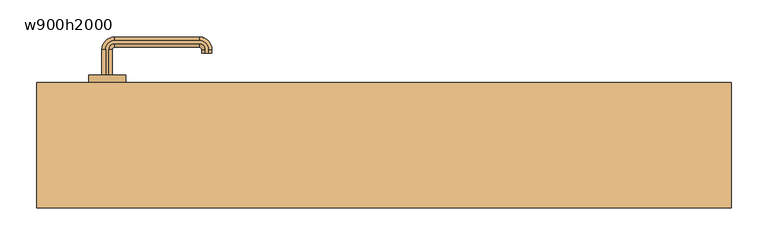
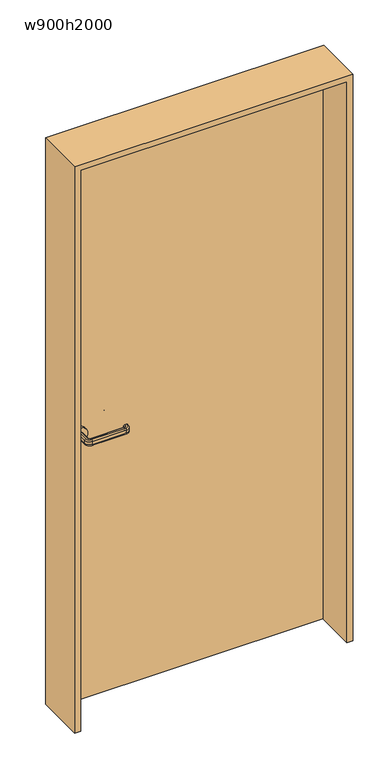
"""IFC4 building model written with IfcOpenShell, lengths in millimetres: door geometry, 片開き : w900h2000."""

from ifc_helpers import new_model, si_unit, point, frame, frame_2d, origin, origin_with_axes, place, context, project, spatial, polyline, circle_curve, ellipse_curve, trimmed, segment, composite_curve, outline, extrude, source, transform, mapped, element, save
from ifc_brep_helpers import plane_surface, cylinder_surface, revolved_surface, advanced_brep


def w900h2000_7a121c74(model_context):
    return source(origin(), model_context, "Body", "SolidModel", [
        advanced_brep(
        [(-377.0, 95.0, 960.0), (-382.0, 95.0, 955.0), (-382.0, 95.0, 945.0477623), (-377.0, 95.0, 940.0477623), (-373.0, 95.0, 940.0477623), (-368.0, 95.0, 945.0477623), (-368.0, 95.0, 955.0), (-373.0, 95.0, 960.0), (-377.0, 130.0, 960.0), (-382.0, 130.0, 955.0), (-382.0, 130.0, 945.0477623), (-377.0, 130.0, 940.0477623), (-365.0, 142.0, 940.0477623), (-250.0, 142.0, 940.0477623), (-238.0, 130.0, 940.0477623), (-238.0, 125.0, 940.0477623), (-242.0, 125.0, 940.0477623), (-242.0, 130.0, 940.0477623), (-250.0, 138.0, 940.0477623), (-365.0, 138.0, 940.0477623), (-373.0, 130.0, 940.0477623), (-368.0, 130.0, 945.0477623), (-368.0, 130.0, 955.0), (-373.0, 130.0, 960.0), (-365.0, 138.0, 960.0), (-250.0, 138.0, 960.0), (-242.0, 130.0, 960.0), (-242.0, 125.0, 960.0), (-238.0, 125.0, 960.0), (-238.0, 130.0, 960.0), (-250.0, 142.0, 960.0), (-365.0, 142.0, 960.0), (-365.0, 147.0, 955.0), (-365.0, 147.0, 945.0477623), (-365.0, 133.0, 945.0477623), (-365.0, 133.0, 955.0), (-250.0, 147.0, 955.0), (-250.0, 147.0, 945.0477623), (-250.0, 133.0, 945.0477623), (-250.0, 133.0, 955.0), (-233.0, 130.0, 955.0), (-233.0, 130.0, 945.0477623), (-247.0, 130.0, 945.0477623), (-247.0, 130.0, 955.0), (-247.0, 125.0, 955.0), (-247.0, 125.0, 945.0477623), (-233.0, 125.0, 945.0477623), (-233.0, 125.0, 955.0)],
        [
            (0, 1, circle_curve(frame((-377.0, 95.0, 955.0), z_axis=(0.0, -1.0, 0.0), x_axis=(-1.0, 0.0, 0.0)), 5.0)),
            (1, 2),
            (2, 3, circle_curve(frame((-377.0, 95.0, 945.0477623), z_axis=(0.0, -1.0, 0.0), x_axis=(-1.0, 0.0, 0.0)), 5.0)),
            (3, 4),
            (4, 5, circle_curve(frame((-373.0, 95.0, 945.0477623), z_axis=(0.0, -1.0, 0.0), x_axis=(-1.0, 0.0, 0.0)), 5.0)),
            (5, 6),
            (6, 7, circle_curve(frame((-373.0, 95.0, 955.0), z_axis=(0.0, -1.0, 0.0), x_axis=(-1.0, 0.0, 0.0)), 5.0)),
            (7, 0),
            (0, 8),
            (8, 9, circle_curve(frame((-377.0, 130.0, 955.0), z_axis=(0.0, -1.0, 0.0), x_axis=(-1.0, 0.0, 0.0)), 5.0)),
            (9, 1),
            (9, 10),
            (10, 2),
            (10, 11, circle_curve(frame((-377.0, 130.0, 945.0477623), z_axis=(0.0, -1.0, 0.0), x_axis=(-1.0, 0.0, 0.0)), 5.0)),
            (11, 3),
            (11, 12, circle_curve(frame((-365.0, 130.0, 940.0477623), z_axis=(0.0, 0.0, -1.0), x_axis=(-1.0, 0.0, 0.0)), 12.0)),
            (12, 13),
            (13, 14, circle_curve(frame((-250.0, 130.0, 940.0477623), z_axis=(0.0, 0.0, -1.0), x_axis=(0.0, 1.0, 0.0)), 12.0)),
            (14, 15),
            (15, 16),
            (16, 17),
            (17, 18, circle_curve(frame((-250.0, 130.0, 940.0477623), z_axis=(0.0, 0.0, 1.0), x_axis=(0.0, 1.0, 0.0)), 8.0)),
            (18, 19),
            (19, 20, circle_curve(frame((-365.0, 130.0, 940.0477623), z_axis=(0.0, 0.0, 1.0), x_axis=(-1.0, 0.0, 0.0)), 8.0)),
            (20, 4),
            (20, 21, circle_curve(frame((-373.0, 130.0, 945.0477623), z_axis=(0.0, -1.0, 0.0), x_axis=(-1.0, 0.0, 0.0)), 5.0)),
            (21, 5),
            (21, 22),
            (22, 6),
            (22, 23, circle_curve(frame((-373.0, 130.0, 955.0), z_axis=(0.0, -1.0, 0.0), x_axis=(-1.0, 0.0, 0.0)), 5.0)),
            (23, 7),
            (23, 24, circle_curve(frame((-365.0, 130.0, 960.0), z_axis=(0.0, 0.0, -1.0), x_axis=(-1.0, 0.0, 0.0)), 8.0)),
            (24, 25),
            (25, 26, circle_curve(frame((-250.0, 130.0, 960.0), z_axis=(0.0, 0.0, -1.0), x_axis=(0.0, 1.0, 0.0)), 8.0)),
            (26, 27),
            (27, 28),
            (28, 29),
            (29, 30, circle_curve(frame((-250.0, 130.0, 960.0), z_axis=(0.0, 0.0, 1.0), x_axis=(0.0, 1.0, 0.0)), 12.0)),
            (30, 31),
            (31, 8, circle_curve(frame((-365.0, 130.0, 960.0), z_axis=(0.0, 0.0, 1.0), x_axis=(-1.0, 0.0, 0.0)), 12.0)),
            (32, 9, circle_curve(frame((-365.0, 130.0, 955.0), z_axis=(0.0, 0.0, 1.0), x_axis=(-1.0, 0.0, 0.0)), 17.0)),
            (31, 32, circle_curve(frame((-365.0, 142.0, 955.0), z_axis=(-1.0, 0.0, 0.0), x_axis=(0.0, 1.0, 0.0)), 5.0)),
            (33, 10, circle_curve(frame((-365.0, 130.0, 945.0477623), z_axis=(0.0, 0.0, 1.0), x_axis=(-1.0, 0.0, 0.0)), 17.0)),
            (32, 33),
            (33, 12, circle_curve(frame((-365.0, 142.0, 945.0477623), z_axis=(-1.0, 0.0, 0.0), x_axis=(0.0, 1.0, 0.0)), 5.0)),
            (34, 21, circle_curve(frame((-365.0, 130.0, 945.0477623), z_axis=(0.0, 0.0, 1.0), x_axis=(-1.0, 0.0, 0.0)), 3.0)),
            (19, 34, circle_curve(frame((-365.0, 138.0, 945.0477623), z_axis=(-1.0, 0.0, 0.0), x_axis=(0.0, 1.0, 0.0)), 5.0)),
            (35, 22, circle_curve(frame((-365.0, 130.0, 955.0), z_axis=(0.0, 0.0, 1.0), x_axis=(-1.0, 0.0, 0.0)), 3.0)),
            (34, 35),
            (35, 24, circle_curve(frame((-365.0, 138.0, 955.0), z_axis=(-1.0, 0.0, 0.0), x_axis=(0.0, 1.0, 0.0)), 5.0)),
            (30, 36, circle_curve(frame((-250.0, 142.0, 955.0), z_axis=(-1.0, 0.0, 0.0), x_axis=(0.0, 1.0, 0.0)), 5.0)),
            (36, 32),
            (36, 37),
            (37, 33),
            (37, 13, circle_curve(frame((-250.0, 142.0, 945.0477623), z_axis=(-1.0, 0.0, 0.0), x_axis=(0.0, 1.0, 0.0)), 5.0)),
            (18, 38, circle_curve(frame((-250.0, 138.0, 945.0477623), z_axis=(-1.0, 0.0, 0.0), x_axis=(0.0, 1.0, 0.0)), 5.0)),
            (38, 34),
            (38, 39),
            (39, 35),
            (39, 25, circle_curve(frame((-250.0, 138.0, 955.0), z_axis=(-1.0, 0.0, 0.0), x_axis=(0.0, 1.0, 0.0)), 5.0)),
            (40, 36, circle_curve(frame((-250.0, 130.0, 955.0), z_axis=(0.0, 0.0, 1.0), x_axis=(0.0, 1.0, 0.0)), 17.0)),
            (29, 40, circle_curve(frame((-238.0, 130.0, 955.0), z_axis=(0.0, 1.0, 0.0), x_axis=(1.0, 0.0, 0.0)), 5.0)),
            (41, 37, circle_curve(frame((-250.0, 130.0, 945.0477623), z_axis=(0.0, 0.0, 1.0), x_axis=(0.0, 1.0, 0.0)), 17.0)),
            (40, 41),
            (41, 14, circle_curve(frame((-238.0, 130.0, 945.0477623), z_axis=(0.0, 1.0, 0.0), x_axis=(1.0, 0.0, 0.0)), 5.0)),
            (42, 38, circle_curve(frame((-250.0, 130.0, 945.0477623), z_axis=(0.0, 0.0, 1.0), x_axis=(0.0, 1.0, 0.0)), 3.0)),
            (17, 42, circle_curve(frame((-242.0, 130.0, 945.0477623), z_axis=(0.0, 1.0, 0.0), x_axis=(1.0, 0.0, 0.0)), 5.0)),
            (43, 39, circle_curve(frame((-250.0, 130.0, 955.0), z_axis=(0.0, 0.0, 1.0), x_axis=(0.0, 1.0, 0.0)), 3.0)),
            (42, 43),
            (43, 26, circle_curve(frame((-242.0, 130.0, 955.0), z_axis=(0.0, 1.0, 0.0), x_axis=(1.0, 0.0, 0.0)), 5.0)),
            (27, 44, circle_curve(frame((-242.0, 125.0, 955.0), z_axis=(0.0, -1.0, 0.0), x_axis=(1.0, 0.0, 0.0)), 5.0)),
            (44, 45),
            (45, 16, circle_curve(frame((-242.0, 125.0, 945.0477623), z_axis=(0.0, -1.0, 0.0), x_axis=(1.0, 0.0, 0.0)), 5.0)),
            (15, 46, circle_curve(frame((-238.0, 125.0, 945.0477623), z_axis=(0.0, -1.0, 0.0), x_axis=(1.0, 0.0, 0.0)), 5.0)),
            (46, 47),
            (47, 28, circle_curve(frame((-238.0, 125.0, 955.0), z_axis=(0.0, -1.0, 0.0), x_axis=(1.0, 0.0, 0.0)), 5.0)),
            (47, 40),
            (46, 41),
            (45, 42),
            (44, 43),
        ],
        [
            plane_surface(frame((-385.198039, 95.0, 950.0), z_axis=(0.0, -1.0, 0.0), x_axis=(0.0, 0.0, 1.0))),
            cylinder_surface(frame((-377.0, 95.0, 955.0), z_axis=(0.0, -1.0, 0.0), x_axis=(-1.0, 0.0, 0.0)), 5.0),
            plane_surface(frame((-382.0, 95.0, 955.0), z_axis=(-1.0, 0.0, 0.0), x_axis=(0.0, 1.0, 0.0))),
            cylinder_surface(frame((-377.0, 95.0, 945.0477623), z_axis=(0.0, -1.0, 0.0), x_axis=(-1.0, 0.0, 0.0)), 5.0),
            plane_surface(frame((-377.0, 95.0, 940.0477623), z_axis=(0.0, 0.0, -1.0), x_axis=(0.0, 1.0, 0.0))),
            cylinder_surface(frame((-373.0, 95.0, 945.0477623), z_axis=(0.0, -1.0, 0.0), x_axis=(-1.0, 0.0, 0.0)), 5.0),
            plane_surface(frame((-368.0, 95.0, 945.0477623), z_axis=(1.0, 0.0, 0.0), x_axis=(0.0, 1.0, 0.0))),
            cylinder_surface(frame((-373.0, 95.0, 955.0), z_axis=(0.0, -1.0, 0.0), x_axis=(-1.0, 0.0, 0.0)), 5.0),
            plane_surface(frame((-373.0, 95.0, 960.0), z_axis=(0.0, 0.0, 1.0), x_axis=(0.0, 1.0, 0.0))),
            revolved_surface(trimmed(ellipse_curve(frame((-377.0, 130.0, 955.0), z_axis=(0.0, -1.0, 0.0), x_axis=(-1.0, 0.0, 0.0)), 5.0, 5.0), [point((-377.0, 130.0, 960.0))], [point((-382.0, 130.0, 955.0))], True, "CARTESIAN"), (-365.0, 130.0, 950.0), (0.0, 0.0, -1.0)),
            cylinder_surface(frame((-365.0, 130.0, 950.0), z_axis=(0.0, 0.0, -1.0), x_axis=(-1.0, 0.0, 0.0)), 17.0),
            revolved_surface(trimmed(ellipse_curve(frame((-377.0, 130.0, 945.0477623), z_axis=(0.0, -1.0, 0.0), x_axis=(-1.0, 0.0, 0.0)), 5.0, 5.0), [point((-382.0, 130.0, 945.0477623))], [point((-377.0, 130.0, 940.0477623))], True, "CARTESIAN"), (-365.0, 130.0, 950.0), (0.0, 0.0, -1.0)),
            revolved_surface(trimmed(ellipse_curve(frame((-373.0, 130.0, 945.0477623), z_axis=(0.0, -1.0, 0.0), x_axis=(-1.0, 0.0, 0.0)), 5.0, 5.0), [point((-373.0, 130.0, 940.0477623))], [point((-368.0, 130.0, 945.0477623))], True, "CARTESIAN"), (-365.0, 130.0, 950.0), (0.0, 0.0, -1.0)),
            revolved_surface(polyline([(-368.0, 130.0, 945.0477623), (-368.0, 130.0, 955.0)]), (-365.0, 130.0, 950.0), (0.0, 0.0, -1.0)),
            revolved_surface(trimmed(ellipse_curve(frame((-373.0, 130.0, 955.0), z_axis=(0.0, -1.0, 0.0), x_axis=(-1.0, 0.0, 0.0)), 5.0, 5.0), [point((-368.0, 130.0, 955.0))], [point((-373.0, 130.0, 960.0))], True, "CARTESIAN"), (-365.0, 130.0, 950.0), (0.0, 0.0, -1.0)),
            cylinder_surface(frame((-365.0, 142.0, 955.0), z_axis=(-1.0, 0.0, 0.0), x_axis=(0.0, 1.0, 0.0)), 5.0),
            plane_surface(frame((-365.0, 147.0, 955.0), z_axis=(0.0, 1.0, 0.0), x_axis=(1.0, 0.0, 0.0))),
            cylinder_surface(frame((-365.0, 142.0, 945.0477623), z_axis=(-1.0, 0.0, 0.0), x_axis=(0.0, 1.0, 0.0)), 5.0),
            cylinder_surface(frame((-365.0, 138.0, 945.0477623), z_axis=(-1.0, 0.0, 0.0), x_axis=(0.0, 1.0, 0.0)), 5.0),
            plane_surface(frame((-365.0, 133.0, 945.0477623), z_axis=(0.0, -1.0, 0.0), x_axis=(1.0, 0.0, 0.0))),
            cylinder_surface(frame((-365.0, 138.0, 955.0), z_axis=(-1.0, 0.0, 0.0), x_axis=(0.0, 1.0, 0.0)), 5.0),
            revolved_surface(trimmed(ellipse_curve(frame((-250.0, 142.0, 955.0), z_axis=(-1.0, 0.0, 0.0), x_axis=(0.0, 1.0, 0.0)), 5.0, 5.0), [point((-250.0, 142.0, 960.0))], [point((-250.0, 147.0, 955.0))], True, "CARTESIAN"), (-250.0, 130.0, 950.0), (0.0, 0.0, -1.0)),
            cylinder_surface(frame((-250.0, 130.0, 950.0), z_axis=(0.0, 0.0, -1.0), x_axis=(0.0, 1.0, 0.0)), 17.0),
            revolved_surface(trimmed(ellipse_curve(frame((-250.0, 142.0, 945.0477623), z_axis=(-1.0, 0.0, 0.0), x_axis=(0.0, 1.0, 0.0)), 5.0, 5.0), [point((-250.0, 147.0, 945.0477623))], [point((-250.0, 142.0, 940.0477623))], True, "CARTESIAN"), (-250.0, 130.0, 950.0), (0.0, 0.0, -1.0)),
            revolved_surface(trimmed(ellipse_curve(frame((-250.0, 138.0, 945.0477623), z_axis=(-1.0, 0.0, 0.0), x_axis=(0.0, 1.0, 0.0)), 5.0, 5.0), [point((-250.0, 138.0, 940.0477623))], [point((-250.0, 133.0, 945.0477623))], True, "CARTESIAN"), (-250.0, 130.0, 950.0), (0.0, 0.0, -1.0)),
            revolved_surface(polyline([(-250.0, 133.0, 945.0477623), (-250.0, 133.0, 955.0)]), (-250.0, 130.0, 950.0), (0.0, 0.0, -1.0)),
            revolved_surface(trimmed(ellipse_curve(frame((-250.0, 138.0, 955.0), z_axis=(-1.0, 0.0, 0.0), x_axis=(0.0, 1.0, 0.0)), 5.0, 5.0), [point((-250.0, 133.0, 955.0))], [point((-250.0, 138.0, 960.0))], True, "CARTESIAN"), (-250.0, 130.0, 950.0), (0.0, 0.0, -1.0)),
            plane_surface(frame((-250.198039, 125.0, 950.0), z_axis=(0.0, -1.0, 0.0), x_axis=(0.0, 0.0, -1.0))),
            cylinder_surface(frame((-238.0, 130.0, 955.0), z_axis=(0.0, 1.0, 0.0), x_axis=(1.0, 0.0, 0.0)), 5.0),
            plane_surface(frame((-233.0, 130.0, 955.0), z_axis=(1.0, 0.0, 0.0), x_axis=(0.0, -1.0, 0.0))),
            cylinder_surface(frame((-238.0, 130.0, 945.0477623), z_axis=(0.0, 1.0, 0.0), x_axis=(1.0, 0.0, 0.0)), 5.0),
            cylinder_surface(frame((-242.0, 130.0, 945.0477623), z_axis=(0.0, 1.0, 0.0), x_axis=(1.0, 0.0, 0.0)), 5.0),
            plane_surface(frame((-247.0, 130.0, 945.0477623), z_axis=(-1.0, 0.0, 0.0), x_axis=(0.0, -1.0, 0.0))),
            cylinder_surface(frame((-242.0, 130.0, 955.0), z_axis=(0.0, 1.0, 0.0), x_axis=(1.0, 0.0, 0.0)), 5.0),
        ],
        [
            (0, [[1, 2, 3, 4, 5, 6, 7, 8]]),
            (1, [[-1, 9, 10, 11]]),
            (2, [[-2, -11, 12, 13]]),
            (3, [[-3, -13, 14, 15]]),
            (4, [[-4, -15, 16, 17, 18, 19, 20, 21, 22, 23, 24, 25]]),
            (5, [[-5, -25, 26, 27]]),
            (6, [[-6, -27, 28, 29]]),
            (7, [[-7, -29, 30, 31]]),
            (8, [[-8, -31, 32, 33, 34, 35, 36, 37, 38, 39, 40, -9]]),
            (9, [[41, -10, -40, 42]]),
            (10, [[43, -12, -41, 44]]),
            (11, [[-16, -14, -43, 45]]),
            (12, [[46, -26, -24, 47]]),
            (13, [[48, -28, -46, 49]]),
            (14, [[-32, -30, -48, 50]]),
            (15, [[-42, -39, 51, 52]]),
            (16, [[-44, -52, 53, 54]]),
            (17, [[-45, -54, 55, -17]]),
            (18, [[-47, -23, 56, 57]]),
            (19, [[-49, -57, 58, 59]]),
            (20, [[-50, -59, 60, -33]]),
            (21, [[61, -51, -38, 62]]),
            (22, [[63, -53, -61, 64]]),
            (23, [[-18, -55, -63, 65]]),
            (24, [[66, -56, -22, 67]]),
            (25, [[68, -58, -66, 69]]),
            (26, [[-34, -60, -68, 70]]),
            (27, [[-36, 71, 72, 73, -20, 74, 75, 76]]),
            (28, [[-62, -37, -76, 77]]),
            (29, [[-64, -77, -75, 78]]),
            (30, [[-65, -78, -74, -19]]),
            (31, [[-67, -21, -73, 79]]),
            (32, [[-69, -79, -72, 80]]),
            (33, [[-70, -80, -71, -35]]),
        ],
    ),
        advanced_brep(
        [(-373.0, 45.0, 940.0), (-377.0, 45.0, 940.0), (-382.0, 45.0, 945.0), (-382.0, 45.0, 955.0), (-377.0, 45.0, 960.0), (-373.0, 45.0, 960.0), (-368.0, 45.0, 955.0), (-368.0, 45.0, 945.0), (-373.0, 10.0, 940.0), (-365.0, 2.0, 940.0), (-250.0, 2.0, 940.0), (-242.0, 10.0, 940.0), (-242.0, 15.0, 940.0), (-238.0, 15.0, 940.0), (-238.0, 10.0, 940.0), (-250.0, -2.0, 940.0), (-365.0, -2.0, 940.0), (-377.0, 10.0, 940.0), (-382.0, 10.0, 945.0), (-382.0, 10.0, 955.0), (-377.0, 10.0, 960.0), (-365.0, -2.0, 960.0), (-250.0, -2.0, 960.0), (-238.0, 10.0, 960.0), (-238.0, 15.0, 960.0), (-242.0, 15.0, 960.0), (-242.0, 10.0, 960.0), (-250.0, 2.0, 960.0), (-365.0, 2.0, 960.0), (-373.0, 10.0, 960.0), (-368.0, 10.0, 955.0), (-368.0, 10.0, 945.0), (-365.0, -7.0, 945.0), (-365.0, -7.0, 955.0), (-365.0, 7.0, 955.0), (-365.0, 7.0, 945.0), (-250.0, -7.0, 945.0), (-250.0, -7.0, 955.0), (-250.0, 7.0, 955.0), (-250.0, 7.0, 945.0), (-233.0, 10.0, 945.0), (-233.0, 10.0, 955.0), (-247.0, 10.0, 955.0), (-247.0, 10.0, 945.0), (-247.0, 15.0, 945.0), (-247.0, 15.0, 955.0), (-233.0, 15.0, 955.0), (-233.0, 15.0, 945.0)],
        [
            (0, 1),
            (1, 2, circle_curve(frame((-377.0, 45.0, 945.0), z_axis=(0.0, 1.0, 0.0), x_axis=(1.0, 0.0, 0.0)), 5.0)),
            (2, 3),
            (3, 4, circle_curve(frame((-377.0, 45.0, 955.0), z_axis=(0.0, 1.0, 0.0), x_axis=(1.0, 0.0, 0.0)), 5.0)),
            (4, 5),
            (5, 6, circle_curve(frame((-373.0, 45.0, 955.0), z_axis=(0.0, 1.0, 0.0), x_axis=(1.0, 0.0, 0.0)), 5.0)),
            (6, 7),
            (7, 0, circle_curve(frame((-373.0, 45.0, 945.0), z_axis=(0.0, 1.0, 0.0), x_axis=(1.0, 0.0, 0.0)), 5.0)),
            (0, 8),
            (8, 9, circle_curve(frame((-365.0, 10.0, 940.0), z_axis=(0.0, 0.0, 1.0), x_axis=(-1.0, 0.0, 0.0)), 8.0)),
            (9, 10),
            (10, 11, circle_curve(frame((-250.0, 10.0, 940.0), z_axis=(0.0, 0.0, 1.0), x_axis=(0.0, -1.0, 0.0)), 8.0)),
            (11, 12),
            (12, 13),
            (13, 14),
            (14, 15, circle_curve(frame((-250.0, 10.0, 940.0), z_axis=(0.0, 0.0, -1.0), x_axis=(0.0, -1.0, 0.0)), 12.0)),
            (15, 16),
            (16, 17, circle_curve(frame((-365.0, 10.0, 940.0), z_axis=(0.0, 0.0, -1.0), x_axis=(-1.0, 0.0, 0.0)), 12.0)),
            (17, 1),
            (17, 18, circle_curve(frame((-377.0, 10.0, 945.0), z_axis=(0.0, 1.0, 0.0), x_axis=(1.0, 0.0, 0.0)), 5.0)),
            (18, 2),
            (18, 19),
            (19, 3),
            (19, 20, circle_curve(frame((-377.0, 10.0, 955.0), z_axis=(0.0, 1.0, 0.0), x_axis=(1.0, 0.0, 0.0)), 5.0)),
            (20, 4),
            (20, 21, circle_curve(frame((-365.0, 10.0, 960.0), z_axis=(0.0, 0.0, 1.0), x_axis=(-1.0, 0.0, 0.0)), 12.0)),
            (21, 22),
            (22, 23, circle_curve(frame((-250.0, 10.0, 960.0), z_axis=(0.0, 0.0, 1.0), x_axis=(0.0, -1.0, 0.0)), 12.0)),
            (23, 24),
            (24, 25),
            (25, 26),
            (26, 27, circle_curve(frame((-250.0, 10.0, 960.0), z_axis=(0.0, 0.0, -1.0), x_axis=(0.0, -1.0, 0.0)), 8.0)),
            (27, 28),
            (28, 29, circle_curve(frame((-365.0, 10.0, 960.0), z_axis=(0.0, 0.0, -1.0), x_axis=(-1.0, 0.0, 0.0)), 8.0)),
            (29, 5),
            (29, 30, circle_curve(frame((-373.0, 10.0, 955.0), z_axis=(0.0, 1.0, 0.0), x_axis=(1.0, 0.0, 0.0)), 5.0)),
            (30, 6),
            (30, 31),
            (31, 7),
            (31, 8, circle_curve(frame((-373.0, 10.0, 945.0), z_axis=(0.0, 1.0, 0.0), x_axis=(1.0, 0.0, 0.0)), 5.0)),
            (32, 18, circle_curve(frame((-365.0, 10.0, 945.0), z_axis=(0.0, 0.0, -1.0), x_axis=(-1.0, 0.0, 0.0)), 17.0)),
            (16, 32, circle_curve(frame((-365.0, -2.0, 945.0), z_axis=(-1.0, 0.0, 0.0), x_axis=(0.0, 1.0, 0.0)), 5.0)),
            (33, 19, circle_curve(frame((-365.0, 10.0, 955.0), z_axis=(0.0, 0.0, -1.0), x_axis=(-1.0, 0.0, 0.0)), 17.0)),
            (32, 33),
            (33, 21, circle_curve(frame((-365.0, -2.0, 955.0), z_axis=(-1.0, 0.0, 0.0), x_axis=(0.0, 1.0, 0.0)), 5.0)),
            (34, 30, circle_curve(frame((-365.0, 10.0, 955.0), z_axis=(0.0, 0.0, -1.0), x_axis=(-1.0, 0.0, 0.0)), 3.0)),
            (28, 34, circle_curve(frame((-365.0, 2.0, 955.0), z_axis=(-1.0, 0.0, 0.0), x_axis=(0.0, 1.0, 0.0)), 5.0)),
            (35, 31, circle_curve(frame((-365.0, 10.0, 945.0), z_axis=(0.0, 0.0, -1.0), x_axis=(-1.0, 0.0, 0.0)), 3.0)),
            (34, 35),
            (35, 9, circle_curve(frame((-365.0, 2.0, 945.0), z_axis=(-1.0, 0.0, 0.0), x_axis=(0.0, 1.0, 0.0)), 5.0)),
            (15, 36, circle_curve(frame((-250.0, -2.0, 945.0), z_axis=(-1.0, 0.0, 0.0), x_axis=(0.0, 1.0, 0.0)), 5.0)),
            (36, 32),
            (36, 37),
            (37, 33),
            (37, 22, circle_curve(frame((-250.0, -2.0, 955.0), z_axis=(-1.0, 0.0, 0.0), x_axis=(0.0, 1.0, 0.0)), 5.0)),
            (27, 38, circle_curve(frame((-250.0, 2.0, 955.0), z_axis=(-1.0, 0.0, 0.0), x_axis=(0.0, 1.0, 0.0)), 5.0)),
            (38, 34),
            (38, 39),
            (39, 35),
            (39, 10, circle_curve(frame((-250.0, 2.0, 945.0), z_axis=(-1.0, 0.0, 0.0), x_axis=(0.0, 1.0, 0.0)), 5.0)),
            (40, 36, circle_curve(frame((-250.0, 10.0, 945.0), z_axis=(0.0, 0.0, -1.0), x_axis=(0.0, -1.0, 0.0)), 17.0)),
            (14, 40, circle_curve(frame((-238.0, 10.0, 945.0), z_axis=(0.0, -1.0, 0.0), x_axis=(-1.0, 0.0, 0.0)), 5.0)),
            (41, 37, circle_curve(frame((-250.0, 10.0, 955.0), z_axis=(0.0, 0.0, -1.0), x_axis=(0.0, -1.0, 0.0)), 17.0)),
            (40, 41),
            (41, 23, circle_curve(frame((-238.0, 10.0, 955.0), z_axis=(0.0, -1.0, 0.0), x_axis=(-1.0, 0.0, 0.0)), 5.0)),
            (42, 38, circle_curve(frame((-250.0, 10.0, 955.0), z_axis=(0.0, 0.0, -1.0), x_axis=(0.0, -1.0, 0.0)), 3.0)),
            (26, 42, circle_curve(frame((-242.0, 10.0, 955.0), z_axis=(0.0, -1.0, 0.0), x_axis=(-1.0, 0.0, 0.0)), 5.0)),
            (43, 39, circle_curve(frame((-250.0, 10.0, 945.0), z_axis=(0.0, 0.0, -1.0), x_axis=(0.0, -1.0, 0.0)), 3.0)),
            (42, 43),
            (43, 11, circle_curve(frame((-242.0, 10.0, 945.0), z_axis=(0.0, -1.0, 0.0), x_axis=(-1.0, 0.0, 0.0)), 5.0)),
            (12, 44, circle_curve(frame((-242.0, 15.0, 945.0), z_axis=(0.0, 1.0, 0.0), x_axis=(-1.0, 0.0, 0.0)), 5.0)),
            (44, 45),
            (45, 25, circle_curve(frame((-242.0, 15.0, 955.0), z_axis=(0.0, 1.0, 0.0), x_axis=(-1.0, 0.0, 0.0)), 5.0)),
            (24, 46, circle_curve(frame((-238.0, 15.0, 955.0), z_axis=(0.0, 1.0, 0.0), x_axis=(-1.0, 0.0, 0.0)), 5.0)),
            (46, 47),
            (47, 13, circle_curve(frame((-238.0, 15.0, 945.0), z_axis=(0.0, 1.0, 0.0), x_axis=(-1.0, 0.0, 0.0)), 5.0)),
            (47, 40),
            (46, 41),
            (45, 42),
            (44, 43),
        ],
        [
            plane_surface(frame((-385.198039, 45.0, 950.0), z_axis=(0.0, 1.0, 0.0), x_axis=(0.0, 0.0, -1.0))),
            plane_surface(frame((-373.0, 45.0, 940.0), z_axis=(0.0, 0.0, -1.0), x_axis=(0.0, -1.0, 0.0))),
            cylinder_surface(frame((-377.0, 45.0, 945.0), z_axis=(0.0, 1.0, 0.0), x_axis=(1.0, 0.0, 0.0)), 5.0),
            plane_surface(frame((-382.0, 45.0, 945.0), z_axis=(-1.0, 0.0, 0.0), x_axis=(0.0, -1.0, 0.0))),
            cylinder_surface(frame((-377.0, 45.0, 955.0), z_axis=(0.0, 1.0, 0.0), x_axis=(1.0, 0.0, 0.0)), 5.0),
            plane_surface(frame((-377.0, 45.0, 960.0), z_axis=(0.0, 0.0, 1.0), x_axis=(0.0, -1.0, 0.0))),
            cylinder_surface(frame((-373.0, 45.0, 955.0), z_axis=(0.0, 1.0, 0.0), x_axis=(1.0, 0.0, 0.0)), 5.0),
            plane_surface(frame((-368.0, 45.0, 955.0), z_axis=(1.0, 0.0, 0.0), x_axis=(0.0, -1.0, 0.0))),
            cylinder_surface(frame((-373.0, 45.0, 945.0), z_axis=(0.0, 1.0, 0.0), x_axis=(1.0, 0.0, 0.0)), 5.0),
            revolved_surface(trimmed(ellipse_curve(frame((-377.0, 10.0, 945.0), z_axis=(0.0, 1.0, 0.0), x_axis=(1.0, 0.0, 0.0)), 5.0, 5.0), [point((-377.0, 10.0, 940.0))], [point((-382.0, 10.0, 945.0))], True, "CARTESIAN"), (-365.0, 10.0, 950.0), (0.0, 0.0, 1.0)),
            cylinder_surface(frame((-365.0, 10.0, 950.0), z_axis=(0.0, 0.0, 1.0), x_axis=(-1.0, 0.0, 0.0)), 17.0),
            revolved_surface(trimmed(ellipse_curve(frame((-377.0, 10.0, 955.0), z_axis=(0.0, 1.0, 0.0), x_axis=(1.0, 0.0, 0.0)), 5.0, 5.0), [point((-382.0, 10.0, 955.0))], [point((-377.0, 10.0, 960.0))], True, "CARTESIAN"), (-365.0, 10.0, 950.0), (0.0, 0.0, 1.0)),
            revolved_surface(trimmed(ellipse_curve(frame((-373.0, 10.0, 955.0), z_axis=(0.0, 1.0, 0.0), x_axis=(1.0, 0.0, 0.0)), 5.0, 5.0), [point((-373.0, 10.0, 960.0))], [point((-368.0, 10.0, 955.0))], True, "CARTESIAN"), (-365.0, 10.0, 950.0), (0.0, 0.0, 1.0)),
            revolved_surface(polyline([(-368.0, 10.0, 955.0), (-368.0, 10.0, 945.0)]), (-365.0, 10.0, 950.0), (0.0, 0.0, 1.0)),
            revolved_surface(trimmed(ellipse_curve(frame((-373.0, 10.0, 945.0), z_axis=(0.0, 1.0, 0.0), x_axis=(1.0, 0.0, 0.0)), 5.0, 5.0), [point((-368.0, 10.0, 945.0))], [point((-373.0, 10.0, 940.0))], True, "CARTESIAN"), (-365.0, 10.0, 950.0), (0.0, 0.0, 1.0)),
            cylinder_surface(frame((-365.0, -2.0, 945.0), z_axis=(-1.0, 0.0, 0.0), x_axis=(0.0, 1.0, 0.0)), 5.0),
            plane_surface(frame((-365.0, -7.0, 945.0), z_axis=(0.0, -1.0, 0.0), x_axis=(1.0, 0.0, 0.0))),
            cylinder_surface(frame((-365.0, -2.0, 955.0), z_axis=(-1.0, 0.0, 0.0), x_axis=(0.0, 1.0, 0.0)), 5.0),
            cylinder_surface(frame((-365.0, 2.0, 955.0), z_axis=(-1.0, 0.0, 0.0), x_axis=(0.0, 1.0, 0.0)), 5.0),
            plane_surface(frame((-365.0, 7.0, 955.0), z_axis=(0.0, 1.0, 0.0), x_axis=(1.0, 0.0, 0.0))),
            cylinder_surface(frame((-365.0, 2.0, 945.0), z_axis=(-1.0, 0.0, 0.0), x_axis=(0.0, 1.0, 0.0)), 5.0),
            revolved_surface(trimmed(ellipse_curve(frame((-250.0, -2.0, 945.0), z_axis=(-1.0, 0.0, 0.0), x_axis=(0.0, 1.0, 0.0)), 5.0, 5.0), [point((-250.0, -2.0, 940.0))], [point((-250.0, -7.0, 945.0))], True, "CARTESIAN"), (-250.0, 10.0, 950.0), (0.0, 0.0, 1.0)),
            cylinder_surface(frame((-250.0, 10.0, 950.0), z_axis=(0.0, 0.0, 1.0), x_axis=(0.0, -1.0, 0.0)), 17.0),
            revolved_surface(trimmed(ellipse_curve(frame((-250.0, -2.0, 955.0), z_axis=(-1.0, 0.0, 0.0), x_axis=(0.0, 1.0, 0.0)), 5.0, 5.0), [point((-250.0, -7.0, 955.0))], [point((-250.0, -2.0, 960.0))], True, "CARTESIAN"), (-250.0, 10.0, 950.0), (0.0, 0.0, 1.0)),
            revolved_surface(trimmed(ellipse_curve(frame((-250.0, 2.0, 955.0), z_axis=(-1.0, 0.0, 0.0), x_axis=(0.0, 1.0, 0.0)), 5.0, 5.0), [point((-250.0, 2.0, 960.0))], [point((-250.0, 7.0, 955.0))], True, "CARTESIAN"), (-250.0, 10.0, 950.0), (0.0, 0.0, 1.0)),
            revolved_surface(polyline([(-250.0, 7.0, 955.0), (-250.0, 7.0, 945.0)]), (-250.0, 10.0, 950.0), (0.0, 0.0, 1.0)),
            revolved_surface(trimmed(ellipse_curve(frame((-250.0, 2.0, 945.0), z_axis=(-1.0, 0.0, 0.0), x_axis=(0.0, 1.0, 0.0)), 5.0, 5.0), [point((-250.0, 7.0, 945.0))], [point((-250.0, 2.0, 940.0))], True, "CARTESIAN"), (-250.0, 10.0, 950.0), (0.0, 0.0, 1.0)),
            plane_surface(frame((-250.198039, 15.0, 950.0), z_axis=(0.0, 1.0, 0.0), x_axis=(0.0, 0.0, 1.0))),
            cylinder_surface(frame((-238.0, 10.0, 945.0), z_axis=(0.0, -1.0, 0.0), x_axis=(-1.0, 0.0, 0.0)), 5.0),
            plane_surface(frame((-233.0, 10.0, 945.0), z_axis=(1.0, 0.0, 0.0), x_axis=(0.0, 1.0, 0.0))),
            cylinder_surface(frame((-238.0, 10.0, 955.0), z_axis=(0.0, -1.0, 0.0), x_axis=(-1.0, 0.0, 0.0)), 5.0),
            cylinder_surface(frame((-242.0, 10.0, 955.0), z_axis=(0.0, -1.0, 0.0), x_axis=(-1.0, 0.0, 0.0)), 5.0),
            plane_surface(frame((-247.0, 10.0, 955.0), z_axis=(-1.0, 0.0, 0.0), x_axis=(0.0, 1.0, 0.0))),
            cylinder_surface(frame((-242.0, 10.0, 945.0), z_axis=(0.0, -1.0, 0.0), x_axis=(-1.0, 0.0, 0.0)), 5.0),
        ],
        [
            (0, [[1, 2, 3, 4, 5, 6, 7, 8]]),
            (1, [[-1, 9, 10, 11, 12, 13, 14, 15, 16, 17, 18, 19]]),
            (2, [[-2, -19, 20, 21]]),
            (3, [[-3, -21, 22, 23]]),
            (4, [[-4, -23, 24, 25]]),
            (5, [[-5, -25, 26, 27, 28, 29, 30, 31, 32, 33, 34, 35]]),
            (6, [[-6, -35, 36, 37]]),
            (7, [[-7, -37, 38, 39]]),
            (8, [[-8, -39, 40, -9]]),
            (9, [[41, -20, -18, 42]]),
            (10, [[43, -22, -41, 44]]),
            (11, [[-26, -24, -43, 45]]),
            (12, [[46, -36, -34, 47]]),
            (13, [[48, -38, -46, 49]]),
            (14, [[-10, -40, -48, 50]]),
            (15, [[-42, -17, 51, 52]]),
            (16, [[-44, -52, 53, 54]]),
            (17, [[-45, -54, 55, -27]]),
            (18, [[-47, -33, 56, 57]]),
            (19, [[-49, -57, 58, 59]]),
            (20, [[-50, -59, 60, -11]]),
            (21, [[61, -51, -16, 62]]),
            (22, [[63, -53, -61, 64]]),
            (23, [[-28, -55, -63, 65]]),
            (24, [[66, -56, -32, 67]]),
            (25, [[68, -58, -66, 69]]),
            (26, [[-12, -60, -68, 70]]),
            (27, [[71, 72, 73, -30, 74, 75, 76, -14]]),
            (28, [[-62, -15, -76, 77]]),
            (29, [[-64, -77, -75, 78]]),
            (30, [[-65, -78, -74, -29]]),
            (31, [[-67, -31, -73, 79]]),
            (32, [[-69, -79, -72, 80]]),
            (33, [[-70, -80, -71, -13]]),
        ],
    ),
        extrude(outline(composite_curve([segment(trimmed(circle_curve(frame_2d((950.0, -375.0)), 25.0), [point((950.0, -400.0))], [point((950.0, -350.0))], False, "CARTESIAN"), True, "CONTINUOUS"), segment(trimmed(circle_curve(frame_2d((950.0, -375.0)), 25.0), [point((950.0, -350.0))], [point((950.0, -400.0))], False, "CARTESIAN"), True, "CONTINUOUS")], self_intersect=False)), frame((0.0, 85.0, 0.0), z_axis=(0.0, 1.0, 0.0), x_axis=(0.0, 0.0, 1.0)), (0.0, 0.0, 1.0), 10.0),
        extrude(outline(composite_curve([segment(trimmed(circle_curve(frame_2d((950.0, -375.0)), 25.0), [point((950.0, -400.0))], [point((950.0, -350.0))], False, "CARTESIAN"), True, "CONTINUOUS"), segment(trimmed(circle_curve(frame_2d((950.0, -375.0)), 25.0), [point((950.0, -350.0))], [point((950.0, -400.0))], False, "CARTESIAN"), True, "CONTINUOUS")], self_intersect=False)), frame((0.0, 45.0, 0.0), z_axis=(0.0, 1.0, 0.0), x_axis=(0.0, 0.0, 1.0)), (0.0, 0.0, 1.0), 10.0),
        extrude(outline(polyline([(2020.0, -470.0), (0.0, -470.0), (0.0, -450.0), (2000.0, -450.0), (2000.0, 450.0), (0.0, 450.0), (0.0, 470.0), (2020.0, 470.0), (2020.0, -470.0)])), frame((0.0, -85.0, 0.0), z_axis=(0.0, 1.0, 0.0), x_axis=(0.0, 0.0, 1.0)), (0.0, 0.0, 1.0), 170.0),
        extrude(outline(polyline([(450.0, 55.0), (-450.0, 55.0), (-450.0, 85.0), (450.0, 85.0), (450.0, 55.0)])), origin_with_axes(), (0.0, 0.0, 1.0), 2000.0),
    ])


if __name__ == "__main__":
    model = new_model("IFC4")
    model_context = context("Model", 3, world=origin())
    ifc_project = project(units=[si_unit("LENGTHUNIT", "METRE", prefix="MILLI")], contexts=[model_context])
    site = spatial("IfcSite", under=ifc_project)
    building = spatial("IfcBuilding", under=site)
    placement = place(None, origin())
    w900h2000_shape = w900h2000_7a121c74(model_context)
    element("IfcDoor", 1, ObjectType="片開き : w900h2000", at=placement, inside=building, context=model_context, shape_type="MappedRepresentation", body=[
        mapped(w900h2000_shape, transform((0.0, 0.0, 0.0), x_axis=(1.0, 0.0, 0.0), y_axis=(0.0, 1.0, 0.0), z_axis=(0.0, 0.0, 1.0))),
    ])
    save(model, "model.ifc")

# Revit data of these elements
# Type "片開き : w900h2000"
#   Construction Type Id = "MDOOR"
#   Analytic Construction = "メタル"
#   Type Mark = "48"
#   Operation = "片側開き戸右"
#   Keynote = "08110.P2"
#   Visual Light Transmittance = 0
#   Solar Heat Gain Coefficient = 0
#   Heat Transfer Coefficient (U) = 3.7021 W/(m²·K)
#   高さ(中心) = 1000 mm
#   Height = 2000 mm
#   Thickness = 30 mm
#   ドア枠見附 = 20 mm
#   Width = 900 mm
#   取手取付け高さ = 950 mm
#   ドア枠ちり = 10 mm
#   Function = 0
#   ドア枠 [instance default] = 塗装ホワイト
#   ドア把手 [instance default] = メタル-ステンレス
#   ドア [instance default] = 塗装ホワイト
#   Wall Closure = (empty or 0)
# Element 1 (IfcDoor, "片開き : w900h2000")
#   Materials on its faces: "メタル-ステンレス", "塗装ホワイト"
# Materials
#   "塗装ホワイト": class "ペイント", colour RGB 249 249 249, transparency 0, Cost = 0
#   "メタル-ステンレス": class "メタル", colour RGB 247 247 247, transparency 0, Cost = 0
